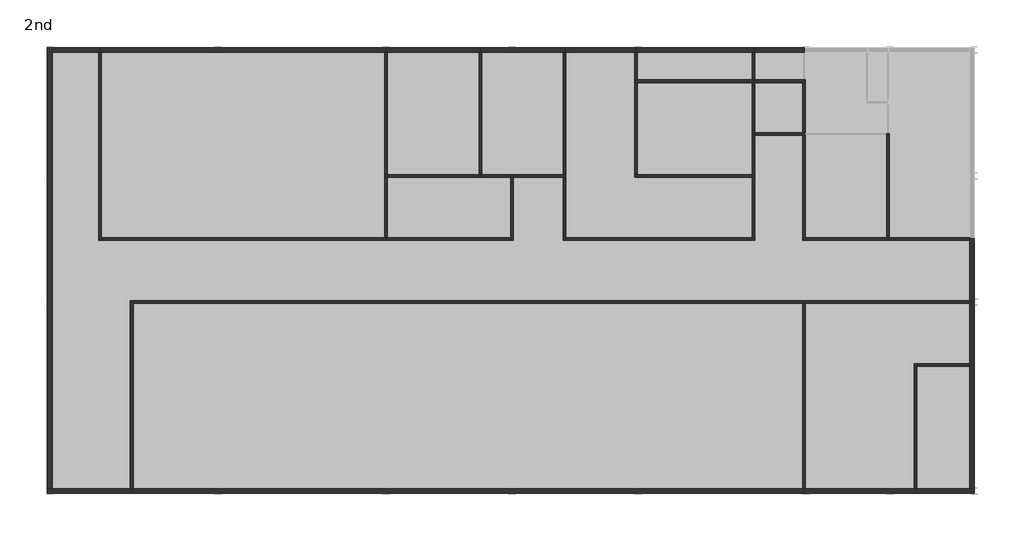
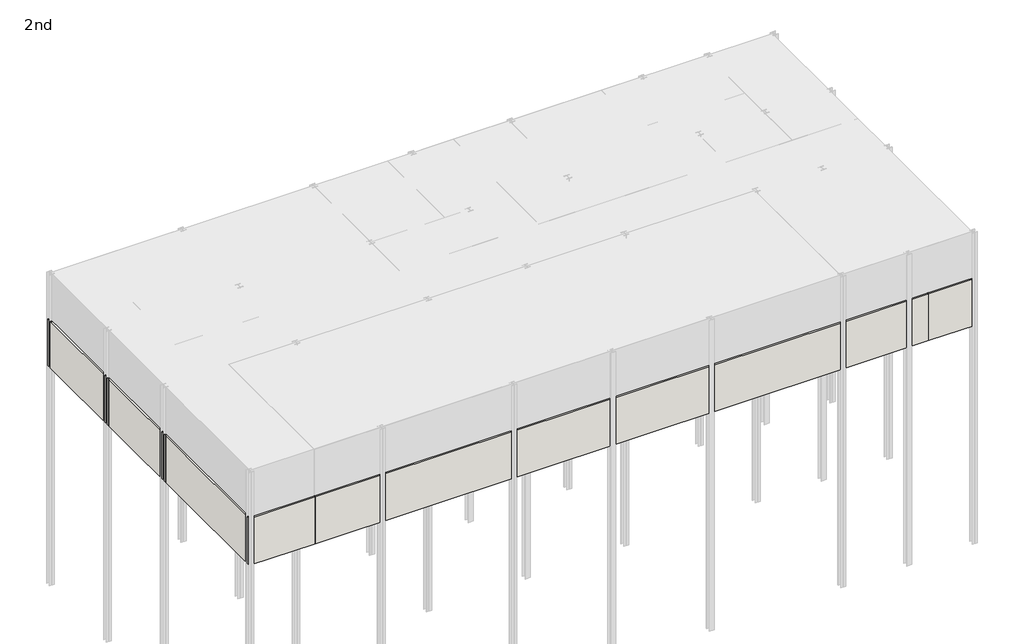
# One storey, part 1 of 3: 49 walls.
"""IFC4 building model written with IfcOpenShell, lengths in millimetres."""

from ifc_helpers import new_model, si_unit, frame, origin, place, context, project, spatial, polyline, outline, extrude, faceted_brep, element, save

model = new_model("IFC4")

# Units and contexts
model_context = context("Model", 3, world=origin())
ifc_project = project(units=[si_unit("LENGTHUNIT", "METRE", prefix="MILLI")], contexts=[model_context])

# Site, building, storey
site = spatial("IfcSite", under=ifc_project)
building = spatial("IfcBuilding", under=site)
storey = spatial("IfcBuildingStorey", under=building, Name="2nd", Elevation=14000.0)

# Walls
placement = place(None, origin())
element("IfcWall", 1, ObjectType="Wall-Ext_215Bwk", at=placement, inside=storey, context=model_context, shape_type="Brep", body=[
    faceted_brep([(160014.1020501, 130908.2581198, 14000.0), (192014.1020501, 130908.2581198, 14000.0), (192014.1020501, 130908.2581198, 17000.0), (160014.1020501, 130908.2581198, 17000.0), (160014.1020501, 131123.2581198, 14000.0), (160014.1020501, 131123.2581198, 17000.0), (160076.6020501, 131123.2581198, 17000.0), (191951.6020501, 131123.2581198, 17000.0), (192014.1020501, 131123.2581198, 17000.0), (192014.1020501, 131123.2581198, 14000.0), (191951.6020501, 131123.2581198, 14000.0), (160076.6020501, 131123.2581198, 14000.0)], [[[0, 1, 2, 3]], [[4, 5, 6, 7, 8, 9, 10, 11]], [[1, 0, 4, 11, 10, 9]], [[2, 1, 9, 8]], [[3, 2, 8, 7, 6, 5]], [[0, 3, 5, 4]]]),
])
element("IfcWall", 2, ObjectType="Wall-Ext_215Bwk", at=placement, inside=storey, context=model_context, shape_type="Brep", body=[
    faceted_brep([(172114.1020501, 152123.2581198, 14000.0), (158514.1020501, 152123.2581198, 14000.0), (158514.1020501, 152123.2581198, 17000.0), (172114.1020501, 152123.2581198, 17000.0), (172114.1020501, 151908.2581198, 14000.0), (172114.1020501, 151908.2581198, 17000.0), (172051.6020501, 151908.2581198, 17000.0), (158576.6020501, 151908.2581198, 17000.0), (158514.1020501, 151908.2581198, 17000.0), (158514.1020501, 151908.2581198, 14000.0), (158576.6020501, 151908.2581198, 14000.0), (172051.6020501, 151908.2581198, 14000.0)], [[[0, 1, 2, 3]], [[4, 5, 6, 7, 8, 9, 10, 11]], [[1, 0, 4, 11, 10, 9]], [[2, 1, 9, 8]], [[3, 2, 8, 7, 6, 5]], [[0, 3, 5, 4]]]),
])
element("IfcWall", 3, ObjectType="Wall-Ext_215Bwk", at=placement, inside=storey, context=model_context, shape_type="Brep", body=[
    faceted_brep([(176614.1020501, 152123.2581198, 14000.0), (172114.1020501, 152123.2581198, 14000.0), (172114.1020501, 152123.2581198, 17000.0), (176614.1020501, 152123.2581198, 17000.0), (176614.1020501, 151908.2581198, 14000.0), (176614.1020501, 151908.2581198, 17000.0), (176551.6020501, 151908.2581198, 17000.0), (172176.6020501, 151908.2581198, 17000.0), (172114.1020501, 151908.2581198, 17000.0), (172114.1020501, 151908.2581198, 14000.0), (172176.6020501, 151908.2581198, 14000.0), (176551.6020501, 151908.2581198, 14000.0)], [[[0, 1, 2, 3]], [[4, 5, 6, 7, 8, 9, 10, 11]], [[1, 0, 4, 11, 10, 9]], [[2, 1, 9, 8]], [[3, 2, 8, 7, 6, 5]], [[0, 3, 5, 4]]]),
])
element("IfcWall", 4, ObjectType="Wall-Ext_215Bwk", at=placement, inside=storey, context=model_context, shape_type="Brep", body=[
    faceted_brep([(180614.1020501, 152123.2581198, 14000.0), (176614.1020501, 152123.2581198, 14000.0), (176614.1020501, 152123.2581198, 17000.0), (180614.1020501, 152123.2581198, 17000.0), (180614.1020501, 151908.2581198, 14000.0), (180614.1020501, 151908.2581198, 17000.0), (180551.6020501, 151908.2581198, 17000.0), (176676.6020501, 151908.2581198, 17000.0), (176614.1020501, 151908.2581198, 17000.0), (176614.1020501, 151908.2581198, 14000.0), (176676.6020501, 151908.2581198, 14000.0), (180551.6020501, 151908.2581198, 14000.0)], [[[0, 1, 2, 3]], [[4, 5, 6, 7, 8, 9, 10, 11]], [[1, 0, 4, 11, 10, 9]], [[2, 1, 9, 8]], [[3, 2, 8, 7, 6, 5]], [[0, 3, 5, 4]]]),
])
element("IfcWall", 5, ObjectType="Wall-Ext_215Bwk", at=placement, inside=storey, context=model_context, shape_type="Brep", body=[
    faceted_brep([(192014.1020501, 152123.2581198, 14000.0), (189614.1020501, 152123.2581198, 14000.0), (189614.1020501, 152123.2581198, 17000.0), (192014.1020501, 152123.2581198, 17000.0), (192014.1020501, 151908.2581198, 14000.0), (192014.1020501, 151908.2581198, 17000.0), (191951.6020501, 151908.2581198, 17000.0), (189676.6020501, 151908.2581198, 17000.0), (189614.1020501, 151908.2581198, 17000.0), (189614.1020501, 151908.2581198, 14000.0), (189676.6020501, 151908.2581198, 14000.0), (191951.6020501, 151908.2581198, 14000.0)], [[[0, 1, 2, 3]], [[4, 5, 6, 7, 8, 9, 10, 11]], [[1, 0, 4, 11, 10, 9]], [[2, 1, 9, 8]], [[3, 2, 8, 7, 6, 5]], [[0, 3, 5, 4]]]),
])
element("IfcWall", 6, ObjectType="Wall-Ext_215Bwk", at=placement, inside=storey, context=model_context, shape_type="Brep", body=[
    faceted_brep([(200121.6020501, 140015.7581198, 14000.0), (200121.6020501, 143015.7581198, 14000.0), (200121.6020501, 143015.7581198, 17000.0), (200121.6020501, 140015.7581198, 17000.0), (199906.6020501, 140015.7581198, 14000.0), (199906.6020501, 140015.7581198, 17000.0), (199906.6020501, 140078.2581198, 17000.0), (199906.6020501, 142953.2581198, 17000.0), (199906.6020501, 143015.7581198, 17000.0), (199906.6020501, 143015.7581198, 14000.0), (199906.6020501, 142953.2581198, 14000.0), (199906.6020501, 140078.2581198, 14000.0)], [[[0, 1, 2, 3]], [[4, 5, 6, 7, 8, 9, 10, 11]], [[1, 0, 4, 11, 10, 9]], [[2, 1, 9, 8]], [[3, 2, 8, 7, 6, 5]], [[0, 3, 5, 4]]]),
])
element("IfcWall", 7, ObjectType="Wall-Ext_215Bwk", at=placement, inside=storey, context=model_context, shape_type="Brep", body=[
    faceted_brep([(158514.1020501, 152123.2581198, 14000.0), (156006.6020501, 152123.2581198, 14000.0), (156006.6020501, 152123.2581198, 17000.0), (158514.1020501, 152123.2581198, 17000.0), (158514.1020501, 151908.2581198, 14000.0), (158514.1020501, 151908.2581198, 17000.0), (158451.6020501, 151908.2581198, 17000.0), (156221.6020501, 151908.2581198, 17000.0), (156006.6020501, 151908.2581198, 17000.0), (156006.6020501, 151908.2581198, 14000.0), (156221.6020501, 151908.2581198, 14000.0), (158451.6020501, 151908.2581198, 14000.0)], [[[0, 1, 2, 3]], [[4, 5, 6, 7, 8, 9, 10, 11]], [[1, 0, 4, 11, 10, 9]], [[3, 2, 8, 7, 6, 5]], [[0, 3, 5, 4]], [[2, 1, 9, 8]]]),
])
element("IfcWall", 8, ObjectType="Wall-Ext_215Bwk", at=placement, inside=storey, context=model_context, shape_type="SweptSolid", body=[
    extrude(outline(polyline([(156006.6020501, 131123.2581198), (156006.6020501, 151908.2581198), (156221.6020501, 151908.2581198), (156221.6020501, 131123.2581198), (156006.6020501, 131123.2581198)])), frame((0.0, 0.0, 14000.0), z_axis=(0.0, 0.0, 1.0), x_axis=(1.0, 0.0, 0.0)), (0.0, 0.0, 1.0), 3000.0),
])
element("IfcWall", 9, ObjectType="Wall-Ext_215Bwk", at=placement, inside=storey, context=model_context, shape_type="Brep", body=[
    faceted_brep([(156006.6020501, 130908.2581198, 14000.0), (160014.1020501, 130908.2581198, 14000.0), (160014.1020501, 130908.2581198, 17000.0), (156006.6020501, 130908.2581198, 17000.0), (156006.6020501, 131123.2581198, 14000.0), (156006.6020501, 131123.2581198, 17000.0), (156221.6020501, 131123.2581198, 17000.0), (159951.6020501, 131123.2581198, 17000.0), (160014.1020501, 131123.2581198, 17000.0), (160014.1020501, 131123.2581198, 14000.0), (159951.6020501, 131123.2581198, 14000.0), (156221.6020501, 131123.2581198, 14000.0)], [[[0, 1, 2, 3]], [[4, 5, 6, 7, 8, 9, 10, 11]], [[1, 0, 4, 11, 10, 9]], [[2, 1, 9, 8]], [[3, 2, 8, 7, 6, 5]], [[0, 3, 5, 4]]]),
])
element("IfcWall", 10, ObjectType="Wall-Ext_215Bwk", at=placement, inside=storey, context=model_context, shape_type="Brep", body=[
    faceted_brep([(189614.1020501, 152123.2581198, 14000.0), (184014.1020501, 152123.2581198, 14000.0), (184014.1020501, 152123.2581198, 17000.0), (189614.1020501, 152123.2581198, 17000.0), (189614.1020501, 151908.2581198, 14000.0), (189614.1020501, 151908.2581198, 17000.0), (189551.6020501, 151908.2581198, 17000.0), (184076.6020501, 151908.2581198, 17000.0), (184014.1020501, 151908.2581198, 17000.0), (184014.1020501, 151908.2581198, 14000.0), (184076.6020501, 151908.2581198, 14000.0), (189551.6020501, 151908.2581198, 14000.0)], [[[0, 1, 2, 3]], [[4, 5, 6, 7, 8, 9, 10, 11]], [[1, 0, 4, 11, 10, 9]], [[2, 1, 9, 8]], [[3, 2, 8, 7, 6, 5]], [[0, 3, 5, 4]]]),
])
element("IfcWall", 11, ObjectType="Wall-Ext_215Bwk", at=placement, inside=storey, context=model_context, shape_type="Brep", body=[
    faceted_brep([(184014.1020501, 152123.2581198, 14000.0), (180614.1020501, 152123.2581198, 14000.0), (180614.1020501, 152123.2581198, 17000.0), (184014.1020501, 152123.2581198, 17000.0), (184014.1020501, 151908.2581198, 14000.0), (184014.1020501, 151908.2581198, 17000.0), (183951.6020501, 151908.2581198, 17000.0), (180676.6020501, 151908.2581198, 17000.0), (180614.1020501, 151908.2581198, 17000.0), (180614.1020501, 151908.2581198, 14000.0), (180676.6020501, 151908.2581198, 14000.0), (183951.6020501, 151908.2581198, 14000.0)], [[[0, 1, 2, 3]], [[4, 5, 6, 7, 8, 9, 10, 11]], [[1, 0, 4, 11, 10, 9]], [[2, 1, 9, 8]], [[3, 2, 8, 7, 6, 5]], [[0, 3, 5, 4]]]),
])
element("IfcWall", 12, ObjectType="Wall-Ext_215Bwk", at=placement, inside=storey, context=model_context, shape_type="Brep", body=[
    faceted_brep([(192014.1020501, 130908.2581198, 14000.0), (197314.1020501, 130908.2581198, 14000.0), (197314.1020501, 130908.2581198, 17000.0), (192014.1020501, 130908.2581198, 17000.0), (192014.1020501, 131123.2581198, 14000.0), (192014.1020501, 131123.2581198, 17000.0), (192076.6020501, 131123.2581198, 17000.0), (197314.1020501, 131123.2581198, 17000.0), (197314.1020501, 131123.2581198, 14000.0), (192076.6020501, 131123.2581198, 14000.0)], [[[0, 1, 2, 3]], [[4, 5, 6, 7, 8, 9]], [[1, 0, 4, 9, 8]], [[2, 1, 8, 7]], [[3, 2, 7, 6, 5]], [[0, 3, 5, 4]]]),
])
element("IfcWall", 13, ObjectType="Wall-Ext_215Bwk", at=placement, inside=storey, context=model_context, shape_type="Brep", body=[
    faceted_brep([(200121.6020501, 137015.7581198, 14000.0), (200121.6020501, 140015.7581198, 14000.0), (200121.6020501, 140015.7581198, 17000.0), (200121.6020501, 137015.7581198, 17000.0), (199906.6020501, 137015.7581198, 14000.0), (199906.6020501, 137015.7581198, 17000.0), (199906.6020501, 137078.2581198, 17000.0), (199906.6020501, 139953.2581198, 17000.0), (199906.6020501, 140015.7581198, 17000.0), (199906.6020501, 140015.7581198, 14000.0), (199906.6020501, 139953.2581198, 14000.0), (199906.6020501, 137078.2581198, 14000.0)], [[[0, 1, 2, 3]], [[4, 5, 6, 7, 8, 9, 10, 11]], [[1, 0, 4, 11, 10, 9]], [[2, 1, 9, 8]], [[3, 2, 8, 7, 6, 5]], [[0, 3, 5, 4]]]),
])
element("IfcWall", 14, ObjectType="Wall-Ext_215Bwk", at=placement, inside=storey, context=model_context, shape_type="Brep", body=[
    faceted_brep([(200121.6020501, 131123.2581198, 14000.0), (200121.6020501, 137015.7581198, 14000.0), (200121.6020501, 137015.7581198, 17000.0), (200121.6020501, 131123.2581198, 17000.0), (199906.6020501, 131123.2581198, 14000.0), (199906.6020501, 131123.2581198, 17000.0), (199906.6020501, 136953.2581198, 17000.0), (199906.6020501, 137015.7581198, 17000.0), (199906.6020501, 137015.7581198, 14000.0), (199906.6020501, 136953.2581198, 14000.0)], [[[0, 1, 2, 3]], [[4, 5, 6, 7, 8, 9]], [[1, 0, 4, 9, 8]], [[2, 1, 8, 7]], [[3, 2, 7, 6, 5]], [[0, 3, 5, 4]]]),
])
element("IfcWall", 15, ObjectType="Wall-Ext_215Bwk", at=placement, inside=storey, context=model_context, shape_type="Brep", body=[
    faceted_brep([(197314.1020501, 130908.2581198, 14000.0), (200121.6020501, 130908.2581198, 14000.0), (200121.6020501, 130908.2581198, 17000.0), (197314.1020501, 130908.2581198, 17000.0), (197314.1020501, 131123.2581198, 14000.0), (197314.1020501, 131123.2581198, 17000.0), (199906.6020501, 131123.2581198, 17000.0), (200121.6020501, 131123.2581198, 17000.0), (200121.6020501, 131123.2581198, 14000.0), (199906.6020501, 131123.2581198, 14000.0)], [[[0, 1, 2, 3]], [[4, 5, 6, 7, 8, 9]], [[1, 0, 4, 9, 8]], [[3, 2, 7, 6, 5]], [[0, 3, 5, 4]], [[2, 1, 8, 7]]]),
])
element("IfcWall", 16, ObjectType="Wall-Int_12P-100Blk-12P", at=placement, inside=storey, context=model_context, shape_type="SweptSolid", body=[
    extrude(outline(polyline([(160076.6020501, 140078.2581198), (191951.6020501, 140078.2581198), (191951.6020501, 139953.2581198), (160076.6020501, 139953.2581198), (160076.6020501, 140078.2581198)])), frame((0.0, 0.0, 14000.0), z_axis=(0.0, 0.0, 1.0), x_axis=(1.0, 0.0, 0.0)), (0.0, 0.0, 1.0), 3000.0),
])
element("IfcWall", 17, ObjectType="Wall-Int_12P-100Blk-12P", at=placement, inside=storey, context=model_context, shape_type="Brep", body=[
    faceted_brep([(159951.6020501, 140078.2581198, 14000.0), (159951.6020501, 131123.2581198, 14000.0), (159951.6020501, 131123.2581198, 17000.0), (159951.6020501, 140078.2581198, 17000.0), (160076.6020501, 140078.2581198, 14000.0), (160076.6020501, 140078.2581198, 17000.0), (160076.6020501, 139953.2581198, 17000.0), (160076.6020501, 131123.2581198, 17000.0), (160076.6020501, 131123.2581198, 14000.0), (160076.6020501, 139953.2581198, 14000.0), (160014.1020501, 131123.2581198, 14000.0), (160014.1020501, 131123.2581198, 17000.0)], [[[0, 1, 2, 3]], [[4, 5, 6, 7, 8, 9]], [[1, 0, 4, 9, 8, 10]], [[3, 2, 11, 7, 6, 5]], [[0, 3, 5, 4]], [[2, 1, 10, 8, 7, 11]]]),
])
element("IfcWall", 18, ObjectType="Wall-Int_12P-100Blk-12P", at=placement, inside=storey, context=model_context, shape_type="Brep", body=[
    faceted_brep([(192076.6020501, 131123.2581198, 14000.0), (192076.6020501, 139953.2581198, 14000.0), (192076.6020501, 140078.2581198, 14000.0), (192076.6020501, 140078.2581198, 17000.0), (192076.6020501, 139953.2581198, 17000.0), (192076.6020501, 131123.2581198, 17000.0), (191951.6020501, 131123.2581198, 14000.0), (191951.6020501, 131123.2581198, 17000.0), (191951.6020501, 139953.2581198, 17000.0), (191951.6020501, 140078.2581198, 17000.0), (191951.6020501, 140078.2581198, 14000.0), (191951.6020501, 139953.2581198, 14000.0), (192014.1020501, 131123.2581198, 14000.0), (192014.1020501, 131123.2581198, 17000.0)], [[[0, 1, 2, 3, 4, 5]], [[6, 7, 8, 9, 10, 11]], [[2, 1, 0, 12, 6, 11, 10]], [[5, 4, 3, 9, 8, 7, 13]], [[3, 2, 10, 9]], [[0, 5, 13, 7, 6, 12]]]),
])
element("IfcWall", 19, ObjectType="Wall-Int_12P-100Blk-12P", at=placement, inside=storey, context=model_context, shape_type="Brep", body=[
    faceted_brep([(158451.6020501, 151908.2581198, 14000.0), (158451.6020501, 142953.2581198, 14000.0), (158451.6020501, 142953.2581198, 17000.0), (158451.6020501, 151908.2581198, 17000.0), (158576.6020501, 151908.2581198, 14000.0), (158576.6020501, 151908.2581198, 17000.0), (158576.6020501, 143078.2581198, 17000.0), (158576.6020501, 142953.2581198, 17000.0), (158576.6020501, 142953.2581198, 14000.0), (158576.6020501, 143078.2581198, 14000.0), (158514.1020501, 151908.2581198, 14000.0), (158514.1020501, 151908.2581198, 17000.0)], [[[0, 1, 2, 3]], [[4, 5, 6, 7, 8, 9]], [[1, 0, 10, 4, 9, 8]], [[3, 2, 7, 6, 5, 11]], [[0, 3, 11, 5, 4, 10]], [[2, 1, 8, 7]]]),
])
element("IfcWall", 20, ObjectType="Wall-Int_12P-100Blk-12P", at=placement, inside=storey, context=model_context, shape_type="Brep", body=[
    faceted_brep([(158576.6020501, 142953.2581198, 14000.0), (172114.1020501, 142953.2581198, 14000.0), (172114.1020501, 142953.2581198, 17000.0), (158576.6020501, 142953.2581198, 17000.0), (158576.6020501, 143078.2581198, 14000.0), (158576.6020501, 143078.2581198, 17000.0), (172051.6020501, 143078.2581198, 17000.0), (172114.1020501, 143078.2581198, 17000.0), (172114.1020501, 143078.2581198, 14000.0), (172051.6020501, 143078.2581198, 14000.0)], [[[0, 1, 2, 3]], [[4, 5, 6, 7, 8, 9]], [[1, 0, 4, 9, 8]], [[2, 1, 8, 7]], [[3, 2, 7, 6, 5]], [[0, 3, 5, 4]]]),
])
element("IfcWall", 21, ObjectType="Wall-Int_12P-100Blk-12P", at=placement, inside=storey, context=model_context, shape_type="Brep", body=[
    faceted_brep([(172176.6020501, 143078.2581198, 14000.0), (172176.6020501, 145953.2581198, 14000.0), (172176.6020501, 145953.2581198, 17000.0), (172176.6020501, 143078.2581198, 17000.0), (172051.6020501, 143078.2581198, 14000.0), (172051.6020501, 143078.2581198, 17000.0), (172051.6020501, 145953.2581198, 17000.0), (172051.6020501, 145953.2581198, 14000.0), (172114.1020501, 143078.2581198, 14000.0), (172114.1020501, 143078.2581198, 17000.0)], [[[0, 1, 2, 3]], [[4, 5, 6, 7]], [[1, 0, 8, 4, 7]], [[3, 2, 6, 5, 9]], [[0, 3, 9, 5, 4, 8]], [[2, 1, 7, 6]]]),
])
element("IfcWall", 22, ObjectType="Wall-Int_12P-100Blk-12P", at=placement, inside=storey, context=model_context, shape_type="Brep", body=[
    faceted_brep([(172176.6020501, 146078.2581198, 14000.0), (172176.6020501, 151908.2581198, 14000.0), (172176.6020501, 151908.2581198, 17000.0), (172176.6020501, 146078.2581198, 17000.0), (172051.6020501, 146078.2581198, 14000.0), (172051.6020501, 146078.2581198, 17000.0), (172051.6020501, 151908.2581198, 17000.0), (172051.6020501, 151908.2581198, 14000.0), (172114.1020501, 151908.2581198, 14000.0), (172114.1020501, 151908.2581198, 17000.0)], [[[0, 1, 2, 3]], [[4, 5, 6, 7]], [[1, 0, 4, 7, 8]], [[3, 2, 9, 6, 5]], [[2, 1, 8, 7, 6, 9]], [[0, 3, 5, 4]]]),
])
element("IfcWall", 23, ObjectType="Wall-Int_12P-100Blk-12P", at=placement, inside=storey, context=model_context, shape_type="Brep", body=[
    faceted_brep([(172051.6020501, 145953.2581198, 14000.0), (172176.6020501, 145953.2581198, 14000.0), (176614.1020501, 145953.2581198, 14000.0), (176614.1020501, 145953.2581198, 17000.0), (172176.6020501, 145953.2581198, 17000.0), (172051.6020501, 145953.2581198, 17000.0), (172051.6020501, 146078.2581198, 14000.0), (172051.6020501, 146078.2581198, 17000.0), (172176.6020501, 146078.2581198, 17000.0), (176551.6020501, 146078.2581198, 17000.0), (176614.1020501, 146078.2581198, 17000.0), (176614.1020501, 146078.2581198, 14000.0), (176551.6020501, 146078.2581198, 14000.0), (172176.6020501, 146078.2581198, 14000.0)], [[[0, 1, 2, 3, 4, 5]], [[6, 7, 8, 9, 10, 11, 12, 13]], [[2, 1, 0, 6, 13, 12, 11]], [[3, 2, 11, 10]], [[5, 4, 3, 10, 9, 8, 7]], [[0, 5, 7, 6]]]),
])
element("IfcWall", 24, ObjectType="Wall-Int_12P-100Blk-12P", at=placement, inside=storey, context=model_context, shape_type="Brep", body=[
    faceted_brep([(176676.6020501, 146078.2581198, 14000.0), (176676.6020501, 151908.2581198, 14000.0), (176676.6020501, 151908.2581198, 17000.0), (176676.6020501, 146078.2581198, 17000.0), (176551.6020501, 146078.2581198, 14000.0), (176551.6020501, 146078.2581198, 17000.0), (176551.6020501, 151908.2581198, 17000.0), (176551.6020501, 151908.2581198, 14000.0), (176614.1020501, 146078.2581198, 14000.0), (176614.1020501, 151908.2581198, 14000.0), (176614.1020501, 151908.2581198, 17000.0), (176614.1020501, 146078.2581198, 17000.0)], [[[0, 1, 2, 3]], [[4, 5, 6, 7]], [[1, 0, 8, 4, 7, 9]], [[3, 2, 10, 6, 5, 11]], [[2, 1, 9, 7, 6, 10]], [[0, 3, 11, 5, 4, 8]]]),
])
element("IfcWall", 25, ObjectType="Wall-Int_12P-100Blk-12P", at=placement, inside=storey, context=model_context, shape_type="Brep", body=[
    faceted_brep([(191951.6020501, 147953.2581198, 14000.0), (191951.6020501, 143078.2581198, 14000.0), (191951.6020501, 143078.2581198, 17000.0), (191951.6020501, 147953.2581198, 17000.0), (192076.6020501, 147953.2581198, 14000.0), (192076.6020501, 147953.2581198, 17000.0), (192076.6020501, 143078.2581198, 17000.0), (192076.6020501, 143078.2581198, 14000.0), (192014.1020501, 147953.2581198, 14000.0), (192014.1020501, 147953.2581198, 17000.0)], [[[0, 1, 2, 3]], [[4, 5, 6, 7]], [[1, 0, 8, 4, 7]], [[3, 2, 6, 5, 9]], [[0, 3, 9, 5, 4, 8]], [[2, 1, 7, 6]]]),
])
element("IfcWall", 26, ObjectType="Wall-Int_12P-100Blk-12P", at=placement, inside=storey, context=model_context, shape_type="Brep", body=[
    faceted_brep([(191951.6020501, 142953.2581198, 14000.0), (196014.1020501, 142953.2581198, 14000.0), (196014.1020501, 142953.2581198, 17000.0), (191951.6020501, 142953.2581198, 17000.0), (191951.6020501, 143078.2581198, 14000.0), (191951.6020501, 143078.2581198, 17000.0), (192076.6020501, 143078.2581198, 17000.0), (195951.6020501, 143078.2581198, 17000.0), (196014.1020501, 143078.2581198, 17000.0), (196014.1020501, 143078.2581198, 14000.0), (195951.6020501, 143078.2581198, 14000.0), (192076.6020501, 143078.2581198, 14000.0)], [[[0, 1, 2, 3]], [[4, 5, 6, 7, 8, 9, 10, 11]], [[1, 0, 4, 11, 10, 9]], [[2, 1, 9, 8]], [[3, 2, 8, 7, 6, 5]], [[0, 3, 5, 4]]]),
])
element("IfcWall", 27, ObjectType="Wall-Int_12P-100Blk-12P", at=placement, inside=storey, context=model_context, shape_type="Brep", body=[
    faceted_brep([(196076.6020501, 143078.2581198, 14000.0), (196076.6020501, 148015.7581198, 14000.0), (196076.6020501, 148015.7581198, 17000.0), (196076.6020501, 143078.2581198, 17000.0), (195951.6020501, 143078.2581198, 14000.0), (195951.6020501, 143078.2581198, 17000.0), (195951.6020501, 147953.2581198, 17000.0), (195951.6020501, 148015.7581198, 17000.0), (195951.6020501, 148015.7581198, 14000.0), (195951.6020501, 147953.2581198, 14000.0), (196014.1020501, 143078.2581198, 14000.0), (196014.1020501, 143078.2581198, 17000.0)], [[[0, 1, 2, 3]], [[4, 5, 6, 7, 8, 9]], [[1, 0, 10, 4, 9, 8]], [[2, 1, 8, 7]], [[3, 2, 7, 6, 5, 11]], [[0, 3, 11, 5, 4, 10]]]),
])
element("IfcWall", 28, ObjectType="Wall-Int_12P-100Blk-12P", at=placement, inside=storey, context=model_context, shape_type="Brep", body=[
    faceted_brep([(196014.1020501, 142953.2581198, 14000.0), (199906.6020501, 142953.2581198, 14000.0), (199906.6020501, 142953.2581198, 17000.0), (196014.1020501, 142953.2581198, 17000.0), (196014.1020501, 143078.2581198, 14000.0), (196014.1020501, 143078.2581198, 17000.0), (196076.6020501, 143078.2581198, 17000.0), (199906.6020501, 143078.2581198, 17000.0), (199906.6020501, 143078.2581198, 14000.0), (196076.6020501, 143078.2581198, 14000.0), (199906.6020501, 143015.7581198, 14000.0), (199906.6020501, 143015.7581198, 17000.0)], [[[0, 1, 2, 3]], [[4, 5, 6, 7, 8, 9]], [[1, 0, 4, 9, 8, 10]], [[3, 2, 11, 7, 6, 5]], [[0, 3, 5, 4]], [[2, 1, 10, 8, 7, 11]]]),
])
element("IfcWall", 29, ObjectType="Wall-Int_12P-100Blk-12P", at=placement, inside=storey, context=model_context, shape_type="Brep", body=[
    faceted_brep([(176614.1020501, 145953.2581198, 14000.0), (178051.6020501, 145953.2581198, 14000.0), (178051.6020501, 145953.2581198, 17000.0), (176614.1020501, 145953.2581198, 17000.0), (176614.1020501, 146078.2581198, 14000.0), (176614.1020501, 146078.2581198, 17000.0), (176676.6020501, 146078.2581198, 17000.0), (178051.6020501, 146078.2581198, 17000.0), (178051.6020501, 146078.2581198, 14000.0), (176676.6020501, 146078.2581198, 14000.0)], [[[0, 1, 2, 3]], [[4, 5, 6, 7, 8, 9]], [[1, 0, 4, 9, 8]], [[3, 2, 7, 6, 5]], [[0, 3, 5, 4]], [[2, 1, 8, 7]]]),
])
element("IfcWall", 30, ObjectType="Wall-Int_12P-100Blk-12P", at=placement, inside=storey, context=model_context, shape_type="Brep", body=[
    faceted_brep([(178176.6020501, 145953.2581198, 14000.0), (180551.6020501, 145953.2581198, 14000.0), (180676.6020501, 145953.2581198, 14000.0), (180676.6020501, 145953.2581198, 17000.0), (180551.6020501, 145953.2581198, 17000.0), (178176.6020501, 145953.2581198, 17000.0), (178176.6020501, 146078.2581198, 14000.0), (178176.6020501, 146078.2581198, 17000.0), (180551.6020501, 146078.2581198, 17000.0), (180676.6020501, 146078.2581198, 17000.0), (180676.6020501, 146078.2581198, 14000.0), (180551.6020501, 146078.2581198, 14000.0)], [[[0, 1, 2, 3, 4, 5]], [[6, 7, 8, 9, 10, 11]], [[2, 1, 0, 6, 11, 10]], [[5, 4, 3, 9, 8, 7]], [[3, 2, 10, 9]], [[0, 5, 7, 6]]]),
])
element("IfcWall", 31, ObjectType="Wall-Int_12P-100Blk-12P", at=placement, inside=storey, context=model_context, shape_type="Brep", body=[
    faceted_brep([(180676.6020501, 146078.2581198, 14000.0), (180676.6020501, 151908.2581198, 14000.0), (180676.6020501, 151908.2581198, 17000.0), (180676.6020501, 146078.2581198, 17000.0), (180551.6020501, 146078.2581198, 14000.0), (180551.6020501, 146078.2581198, 17000.0), (180551.6020501, 151908.2581198, 17000.0), (180551.6020501, 151908.2581198, 14000.0), (180614.1020501, 151908.2581198, 14000.0), (180614.1020501, 151908.2581198, 17000.0)], [[[0, 1, 2, 3]], [[4, 5, 6, 7]], [[1, 0, 4, 7, 8]], [[3, 2, 9, 6, 5]], [[2, 1, 8, 7, 6, 9]], [[0, 3, 5, 4]]]),
])
element("IfcWall", 32, ObjectType="Wall-Int_12P-100Blk-12P", at=placement, inside=storey, context=model_context, shape_type="Brep", body=[
    faceted_brep([(172114.1020501, 142953.2581198, 14000.0), (178051.6020501, 142953.2581198, 14000.0), (178051.6020501, 142953.2581198, 17000.0), (172114.1020501, 142953.2581198, 17000.0), (172114.1020501, 143078.2581198, 14000.0), (172114.1020501, 143078.2581198, 17000.0), (172176.6020501, 143078.2581198, 17000.0), (178051.6020501, 143078.2581198, 17000.0), (178051.6020501, 143078.2581198, 14000.0), (172176.6020501, 143078.2581198, 14000.0)], [[[0, 1, 2, 3]], [[4, 5, 6, 7, 8, 9]], [[1, 0, 4, 9, 8]], [[3, 2, 7, 6, 5]], [[0, 3, 5, 4]], [[2, 1, 8, 7]]]),
])
element("IfcWall", 33, ObjectType="Wall-Int_12P-100Blk-12P", at=placement, inside=storey, context=model_context, shape_type="Brep", body=[
    faceted_brep([(178176.6020501, 142953.2581198, 14000.0), (178176.6020501, 145953.2581198, 14000.0), (178176.6020501, 146078.2581198, 14000.0), (178176.6020501, 146078.2581198, 17000.0), (178176.6020501, 145953.2581198, 17000.0), (178176.6020501, 142953.2581198, 17000.0), (178051.6020501, 142953.2581198, 14000.0), (178051.6020501, 142953.2581198, 17000.0), (178051.6020501, 143078.2581198, 17000.0), (178051.6020501, 145953.2581198, 17000.0), (178051.6020501, 146078.2581198, 17000.0), (178051.6020501, 146078.2581198, 14000.0), (178051.6020501, 145953.2581198, 14000.0), (178051.6020501, 143078.2581198, 14000.0)], [[[0, 1, 2, 3, 4, 5]], [[6, 7, 8, 9, 10, 11, 12, 13]], [[2, 1, 0, 6, 13, 12, 11]], [[5, 4, 3, 10, 9, 8, 7]], [[0, 5, 7, 6]], [[3, 2, 11, 10]]]),
])
element("IfcWall", 34, ObjectType="Wall-Int_12P-100Blk-12P", at=placement, inside=storey, context=model_context, shape_type="Brep", body=[
    faceted_brep([(189551.6020501, 151908.2581198, 14000.0), (189551.6020501, 150578.2581198, 14000.0), (189551.6020501, 150578.2581198, 17000.0), (189551.6020501, 151908.2581198, 17000.0), (189676.6020501, 151908.2581198, 14000.0), (189676.6020501, 151908.2581198, 17000.0), (189676.6020501, 150578.2581198, 17000.0), (189676.6020501, 150578.2581198, 14000.0), (189614.1020501, 151908.2581198, 14000.0), (189614.1020501, 150578.2581198, 14000.0), (189614.1020501, 150578.2581198, 17000.0), (189614.1020501, 151908.2581198, 17000.0)], [[[0, 1, 2, 3]], [[4, 5, 6, 7]], [[1, 0, 8, 4, 7, 9]], [[3, 2, 10, 6, 5, 11]], [[0, 3, 11, 5, 4, 8]], [[2, 1, 9, 7, 6, 10]]]),
])
element("IfcWall", 35, ObjectType="Wall-Int_12P-100Blk-12P", at=placement, inside=storey, context=model_context, shape_type="Brep", body=[
    faceted_brep([(189614.1020501, 150453.2581198, 14000.0), (189676.6020501, 150453.2581198, 14000.0), (191951.6020501, 150453.2581198, 14000.0), (192076.6020501, 150453.2581198, 14000.0), (192076.6020501, 150453.2581198, 17000.0), (191951.6020501, 150453.2581198, 17000.0), (189676.6020501, 150453.2581198, 17000.0), (189614.1020501, 150453.2581198, 17000.0), (189614.1020501, 150578.2581198, 14000.0), (189614.1020501, 150578.2581198, 17000.0), (189676.6020501, 150578.2581198, 17000.0), (191951.6020501, 150578.2581198, 17000.0), (192076.6020501, 150578.2581198, 17000.0), (192076.6020501, 150578.2581198, 14000.0), (191951.6020501, 150578.2581198, 14000.0), (189676.6020501, 150578.2581198, 14000.0)], [[[0, 1, 2, 3, 4, 5, 6, 7]], [[8, 9, 10, 11, 12, 13, 14, 15]], [[3, 2, 1, 0, 8, 15, 14, 13]], [[7, 6, 5, 4, 12, 11, 10, 9]], [[0, 7, 9, 8]], [[4, 3, 13, 12]]]),
])
element("IfcWall", 36, ObjectType="Wall-Int_12P-100Blk-12P", at=placement, inside=storey, context=model_context, shape_type="Brep", body=[
    faceted_brep([(192076.6020501, 139953.2581198, 14000.0), (199906.6020501, 139953.2581198, 14000.0), (199906.6020501, 139953.2581198, 17000.0), (192076.6020501, 139953.2581198, 17000.0), (192076.6020501, 140078.2581198, 14000.0), (192076.6020501, 140078.2581198, 17000.0), (199906.6020501, 140078.2581198, 17000.0), (199906.6020501, 140078.2581198, 14000.0), (199906.6020501, 140015.7581198, 14000.0), (199906.6020501, 140015.7581198, 17000.0)], [[[0, 1, 2, 3]], [[4, 5, 6, 7]], [[1, 0, 4, 7, 8]], [[3, 2, 9, 6, 5]], [[0, 3, 5, 4]], [[2, 1, 8, 7, 6, 9]]]),
])
element("IfcWall", 37, ObjectType="Wall-Int_12P-100Blk-12P", at=placement, inside=storey, context=model_context, shape_type="Brep", body=[
    faceted_brep([(192014.1020501, 148078.2581198, 14000.0), (191951.6020501, 148078.2581198, 14000.0), (189614.1020501, 148078.2581198, 14000.0), (189614.1020501, 148078.2581198, 17000.0), (191951.6020501, 148078.2581198, 17000.0), (192014.1020501, 148078.2581198, 17000.0), (192014.1020501, 147953.2581198, 14000.0), (192014.1020501, 147953.2581198, 17000.0), (191951.6020501, 147953.2581198, 17000.0), (189614.1020501, 147953.2581198, 17000.0), (189614.1020501, 147953.2581198, 14000.0), (191951.6020501, 147953.2581198, 14000.0)], [[[0, 1, 2, 3, 4, 5]], [[6, 7, 8, 9, 10, 11]], [[2, 1, 0, 6, 11, 10]], [[3, 2, 10, 9]], [[5, 4, 3, 9, 8, 7]], [[0, 5, 7, 6]]]),
])
element("IfcWall", 38, ObjectType="Wall-Int_12P-100Blk-12P", at=placement, inside=storey, context=model_context, shape_type="SweptSolid", body=[
    extrude(outline(polyline([(189551.6020501, 146015.7581198), (189551.6020501, 148015.7581198), (189676.6020501, 148015.7581198), (189676.6020501, 146015.7581198), (189551.6020501, 146015.7581198)])), frame((0.0, 0.0, 14000.0), z_axis=(0.0, 0.0, 1.0), x_axis=(1.0, 0.0, 0.0)), (0.0, 0.0, 1.0), 3000.0),
])
element("IfcWall", 39, ObjectType="Wall-Int_12P-100Blk-12P", at=placement, inside=storey, context=model_context, shape_type="SweptSolid", body=[
    extrude(outline(polyline([(189551.6020501, 143078.2581198), (189551.6020501, 146015.7581198), (189676.6020501, 146015.7581198), (189676.6020501, 143078.2581198), (189551.6020501, 143078.2581198)])), frame((0.0, 0.0, 14000.0), z_axis=(0.0, 0.0, 1.0), x_axis=(1.0, 0.0, 0.0)), (0.0, 0.0, 1.0), 3000.0),
])
element("IfcWall", 40, ObjectType="Wall-Int_12P-100Blk-12P", at=placement, inside=storey, context=model_context, shape_type="Brep", body=[
    faceted_brep([(189676.6020501, 143078.2581198, 14000.0), (189551.6020501, 143078.2581198, 14000.0), (180676.6020501, 143078.2581198, 14000.0), (180551.6020501, 143078.2581198, 14000.0), (180551.6020501, 143078.2581198, 17000.0), (180676.6020501, 143078.2581198, 17000.0), (189551.6020501, 143078.2581198, 17000.0), (189676.6020501, 143078.2581198, 17000.0), (189676.6020501, 142953.2581198, 14000.0), (189676.6020501, 142953.2581198, 17000.0), (180551.6020501, 142953.2581198, 17000.0), (180551.6020501, 142953.2581198, 14000.0)], [[[0, 1, 2, 3, 4, 5, 6, 7]], [[8, 9, 10, 11]], [[3, 2, 1, 0, 8, 11]], [[7, 6, 5, 4, 10, 9]], [[0, 7, 9, 8]], [[4, 3, 11, 10]]]),
])
element("IfcWall", 41, ObjectType="Wall-Int_12P-100Blk-12P", at=placement, inside=storey, context=model_context, shape_type="SweptSolid", body=[
    extrude(outline(polyline([(180676.6020501, 145953.2581198), (180676.6020501, 143078.2581198), (180551.6020501, 143078.2581198), (180551.6020501, 145953.2581198), (180676.6020501, 145953.2581198)])), frame((0.0, 0.0, 14000.0), z_axis=(0.0, 0.0, 1.0), x_axis=(1.0, 0.0, 0.0)), (0.0, 0.0, 1.0), 3000.0),
])
element("IfcWall", 42, ObjectType="Wall-Int_12P-100Blk-12P", at=placement, inside=storey, context=model_context, shape_type="Brep", body=[
    faceted_brep([(189551.6020501, 150453.2581198, 14000.0), (189551.6020501, 148015.7581198, 14000.0), (189551.6020501, 148015.7581198, 17000.0), (189551.6020501, 150453.2581198, 17000.0), (189676.6020501, 150453.2581198, 14000.0), (189676.6020501, 150453.2581198, 17000.0), (189676.6020501, 148015.7581198, 17000.0), (189676.6020501, 148015.7581198, 14000.0), (189614.1020501, 150453.2581198, 14000.0), (189614.1020501, 150453.2581198, 17000.0)], [[[0, 1, 2, 3]], [[4, 5, 6, 7]], [[1, 0, 8, 4, 7]], [[2, 1, 7, 6]], [[3, 2, 6, 5, 9]], [[0, 3, 9, 5, 4, 8]]]),
])
element("IfcWall", 43, ObjectType="Wall-Int_12P-100Blk-12P", at=placement, inside=storey, context=model_context, shape_type="Brep", body=[
    faceted_brep([(192076.6020501, 148078.2581198, 14000.0), (192076.6020501, 150453.2581198, 14000.0), (192076.6020501, 150453.2581198, 17000.0), (192076.6020501, 148078.2581198, 17000.0), (191951.6020501, 148078.2581198, 14000.0), (191951.6020501, 148078.2581198, 17000.0), (191951.6020501, 150453.2581198, 17000.0), (191951.6020501, 150453.2581198, 14000.0), (192014.1020501, 148078.2581198, 14000.0), (192014.1020501, 148078.2581198, 17000.0)], [[[0, 1, 2, 3]], [[4, 5, 6, 7]], [[1, 0, 8, 4, 7]], [[3, 2, 6, 5, 9]], [[0, 3, 9, 5, 4, 8]], [[2, 1, 7, 6]]]),
])
element("IfcWall", 44, ObjectType="Wall-Int_12P-100Blk-12P", at=placement, inside=storey, context=model_context, shape_type="Brep", body=[
    faceted_brep([(183951.6020501, 151908.2581198, 14000.0), (183951.6020501, 150578.2581198, 14000.0), (183951.6020501, 150578.2581198, 17000.0), (183951.6020501, 151908.2581198, 17000.0), (184076.6020501, 151908.2581198, 14000.0), (184076.6020501, 151908.2581198, 17000.0), (184076.6020501, 150578.2581198, 17000.0), (184076.6020501, 150578.2581198, 14000.0), (184014.1020501, 151908.2581198, 14000.0), (184014.1020501, 151908.2581198, 17000.0)], [[[0, 1, 2, 3]], [[4, 5, 6, 7]], [[1, 0, 8, 4, 7]], [[3, 2, 6, 5, 9]], [[0, 3, 9, 5, 4, 8]], [[2, 1, 7, 6]]]),
])
element("IfcWall", 45, ObjectType="Wall-Int_12P-100Blk-12P", at=placement, inside=storey, context=model_context, shape_type="Brep", body=[
    faceted_brep([(183951.6020501, 150453.2581198, 14000.0), (184076.6020501, 150453.2581198, 14000.0), (189551.6020501, 150453.2581198, 14000.0), (189614.1020501, 150453.2581198, 14000.0), (189614.1020501, 150453.2581198, 17000.0), (189551.6020501, 150453.2581198, 17000.0), (184076.6020501, 150453.2581198, 17000.0), (183951.6020501, 150453.2581198, 17000.0), (183951.6020501, 150578.2581198, 14000.0), (183951.6020501, 150578.2581198, 17000.0), (184076.6020501, 150578.2581198, 17000.0), (189551.6020501, 150578.2581198, 17000.0), (189614.1020501, 150578.2581198, 17000.0), (189614.1020501, 150578.2581198, 14000.0), (189551.6020501, 150578.2581198, 14000.0), (184076.6020501, 150578.2581198, 14000.0)], [[[0, 1, 2, 3, 4, 5, 6, 7]], [[8, 9, 10, 11, 12, 13, 14, 15]], [[3, 2, 1, 0, 8, 15, 14, 13]], [[4, 3, 13, 12]], [[7, 6, 5, 4, 12, 11, 10, 9]], [[0, 7, 9, 8]]]),
])
element("IfcWall", 46, ObjectType="Wall-Int_12P-100Blk-12P", at=placement, inside=storey, context=model_context, shape_type="Brep", body=[
    faceted_brep([(189614.1020501, 146078.2581198, 14000.0), (184076.6020501, 146078.2581198, 14000.0), (183951.6020501, 146078.2581198, 14000.0), (183951.6020501, 146078.2581198, 17000.0), (184076.6020501, 146078.2581198, 17000.0), (189614.1020501, 146078.2581198, 17000.0), (189614.1020501, 145953.2581198, 14000.0), (189614.1020501, 145953.2581198, 17000.0), (183951.6020501, 145953.2581198, 17000.0), (183951.6020501, 145953.2581198, 14000.0)], [[[0, 1, 2, 3, 4, 5]], [[6, 7, 8, 9]], [[2, 1, 0, 6, 9]], [[5, 4, 3, 8, 7]], [[0, 5, 7, 6]], [[3, 2, 9, 8]]]),
])
element("IfcWall", 47, ObjectType="Wall-Int_12P-100Blk-12P", at=placement, inside=storey, context=model_context, shape_type="SweptSolid", body=[
    extrude(outline(polyline([(184076.6020501, 150453.2581198), (184076.6020501, 146078.2581198), (183951.6020501, 146078.2581198), (183951.6020501, 150453.2581198), (184076.6020501, 150453.2581198)])), frame((0.0, 0.0, 14000.0), z_axis=(0.0, 0.0, 1.0), x_axis=(1.0, 0.0, 0.0)), (0.0, 0.0, 1.0), 3000.0),
])
element("IfcWall", 48, ObjectType="Wall-Int_12P-100Blk-12P", at=placement, inside=storey, context=model_context, shape_type="SweptSolid", body=[
    extrude(outline(polyline([(197376.6020501, 136953.2581198), (197376.6020501, 131015.7581198), (197251.6020501, 131015.7581198), (197251.6020501, 136953.2581198), (197376.6020501, 136953.2581198)])), frame((0.0, 0.0, 14000.0), z_axis=(0.0, 0.0, 1.0), x_axis=(1.0, 0.0, 0.0)), (0.0, 0.0, 1.0), 3000.0),
])
element("IfcWall", 49, ObjectType="Wall-Int_12P-100Blk-12P", at=placement, inside=storey, context=model_context, shape_type="Brep", body=[
    faceted_brep([(197251.6020501, 136953.2581198, 14000.0), (197376.6020501, 136953.2581198, 14000.0), (199906.6020501, 136953.2581198, 14000.0), (199906.6020501, 136953.2581198, 17000.0), (197376.6020501, 136953.2581198, 17000.0), (197251.6020501, 136953.2581198, 17000.0), (197251.6020501, 137078.2581198, 14000.0), (197251.6020501, 137078.2581198, 17000.0), (199906.6020501, 137078.2581198, 17000.0), (199906.6020501, 137078.2581198, 14000.0), (199906.6020501, 137015.7581198, 14000.0), (199906.6020501, 137015.7581198, 17000.0)], [[[0, 1, 2, 3, 4, 5]], [[6, 7, 8, 9]], [[2, 1, 0, 6, 9, 10]], [[5, 4, 3, 11, 8, 7]], [[0, 5, 7, 6]], [[3, 2, 10, 9, 8, 11]]]),
])

save(model, "model.ifc")

# Revit data of these elements
# Project information
#   Project Issue Date = "Issue Date"
#   Project Status = "Project Status"
#   Client Name = "Owner"
#   Project Address = "Enter address here"
#   Project Name = "Project Name"
#   Project Number = "Project Number"
# Grids (mm)
#   "A": line (156114.102, 123537.292) -> (156114.102, 157930.913)
#   "B": line (164114.102, 123537.292) -> (164114.102, 157930.913)
#   "C": line (172114.102, 123537.292) -> (172114.102, 157930.913)
#   "D": line (178114.102, 123537.292) -> (178114.102, 157930.913)
#   "E": line (184114.102, 123537.292) -> (184114.102, 157930.913)
#   "F": line (192114.102, 123537.292) -> (192114.102, 157930.913)
#   "G": line (196114.102, 123537.292) -> (196114.102, 157930.913)
#   "8": line (145724.678, 152015.758) -> (209069.776, 152015.758)
#   "3": line (145724.678, 146015.758) -> (209069.776, 146015.758)
#   "2": line (145724.678, 140015.758) -> (209069.776, 140015.758)
#   "1": line (145724.678, 131015.758) -> (209069.776, 131015.758)
#   "H": line (200114.102, 123537.292) -> (200114.102, 157930.913)
# Type "Wall-Ext_215Bwk"
#   Keynote = "F10"
#   Layers, outside or top first: 215 mm "Brick, Common" (function 1)
# Type "Wall-Int_12P-100Blk-12P"
#   Layers, outside or top first: 12.5 mm "Plaster" (function 5); 100 mm "Concrete Masonry Units" (function 1); 12.5 mm "Plaster" (function 5)
# Elements 1, 2, 3, 4, 5, 6, 7, 8, 9, 10, 11, 12, 13, 14, 15 (IfcWall, "Wall-Ext_215Bwk")
#   Top Offset = 0 mm
#   Base Offset = 0 mm
#   Unconnected Height = 3000 mm
#   wall height = 3000 mm
#   Phase Created = New Construction
#   Base Constraint = 2nd
#   Materials on its faces: "Brick, Common"
# Elements 16, 20, 21, 22, 24, 25, 27, 28, 29, 31, 32, 34, 36, 37, 38, 39, 41, 42, 43, 44, 47, 48 (IfcWall, "Wall-Int_12P-100Blk-12P")
#   Top Offset = 0 mm
#   Base Offset = 0 mm
#   Unconnected Height = 3000 mm
#   wall height = 3000 mm
#   Phase Created = New Construction
#   Base Constraint = 2nd
#   Materials on its faces: "Default Wall", "Plaster"
# Elements 17, 18, 19, 23, 26, 30, 33, 35, 40, 45, 46, 49 (IfcWall, "Wall-Int_12P-100Blk-12P")
#   Top Offset = 0 mm
#   Base Offset = 0 mm
#   Unconnected Height = 3000 mm
#   wall height = 3000 mm
#   Phase Created = New Construction
#   Base Constraint = 2nd
#   Materials on its faces: "Plaster", "Default Wall"
# Materials
#   "Brick, Common": class "Masonry", colour RGB 170 100 105, transparency 0, Description = "Common brick", Cost = 0
#   "Plaster": class "Generic", colour RGB 249 249 249, transparency 0, Description = "Plaster", Cost = 0
#   "Concrete Masonry Units": class "Masonry", colour RGB 181 181 181, transparency 0, Description = "Concrete masonry units", Cost = 0
#   "Default Wall": class "Miscellaneous", colour RGB 128 128 128, transparency 0, Comments = "Rendering appearance not upgraded Rendering appearance not upgraded ", Cost = 0
# Room at (176014.102, 135515.758) mm, phase "New Construction", upper offset 2438.4 mm, lower offset 0 mm
#   Department = "CI"
#   Number = "3.0"
#   Name = "Central Control Room"
#   Interior Finish = "IF3"
#   Exterior Finish = "EF1"
# Room at (165314.102, 147515.758) mm, phase "New Construction", upper offset 2438.4 mm, lower offset 0 mm
#   Department = "CI"
#   Number = "3.1"
#   Name = "Engineer Room"
#   Interior Finish = "IF3"
#   Exterior Finish = "EF1"
# Room at (174364.102, 149015.758) mm, phase "New Construction", upper offset 2438.4 mm, lower offset 0 mm
#   Department = "AR"
#   Number = "3.2"
#   Name = "Document Room"
#   Interior Finish = "IF2-1"
#   Exterior Finish = "EF1"
# Room at (194014.102, 145515.758) mm, phase "New Construction", upper offset 2438.4 mm, lower offset 0 mm
#   Department = "AR"
#   Number = "3.3"
#   Name = "Toilet (M)"
#   Interior Finish = "IF5"
#   Exterior Finish = "EF1"
# Room at (198014.102, 147515.758) mm, phase "New Construction", upper offset 2438.4 mm, lower offset 0 mm
#   Department = "AR"
#   Number = "3.4"
#   Name = "Stairway"
#   Interior Finish = "IF2"
#   Exterior Finish = "EF1"
# Room at (178614.102, 149015.758) mm, phase "New Construction", upper offset 2438.4 mm, lower offset 0 mm
#   Number = "3.5"
#   Name = "Shift Office Room"
# Room at (175114.102, 144515.758) mm, phase "New Construction", upper offset 2438.4 mm, lower offset 0 mm
#   Department = "AR"
#   Number = "3.6"
#   Name = "LOTO Office Room"
#   Interior Finish = "IF2-1"
#   Exterior Finish = "EF1"
# Room at (190814.102, 151265.758) mm, phase "New Construction", upper offset 2438.4 mm, lower offset 0 mm
#   Number = "3.7"
#   Name = "Shower Room (F)"
# Room at (178064.102, 141515.758) mm, phase "New Construction", upper offset 2438.4 mm, lower offset 0 mm
#   Department = "AR"
#   Number = "3.8"
#   Name = "Corridor"
#   Interior Finish = "IF2-1"
#   Exterior Finish = "EF1"
# Room at (190814.102, 149265.758) mm, phase "New Construction", upper offset 2438.4 mm, lower offset 0 mm
#   Number = "3.9"
#   Name = "Locker Room (F)"
# Room at (186814.102, 148265.758) mm, phase "New Construction", upper offset 2438.4 mm, lower offset 0 mm
#   Department = "AR"
#   Number = "3.12"
#   Name = "Locker Room (M)"
#   Interior Finish = "IF2-1"
#   Exterior Finish = "EF1"
# Room at (196014.102, 135515.758) mm, phase "New Construction", upper offset 2438.4 mm, lower offset 0 mm
#   Department = "HV"
#   Number = "3.13"
#   Name = "Duct Shaft"
#   Interior Finish = "NA"
#   Exterior Finish = "EF1"
# Room at (198664.102, 134015.758) mm, phase "New Construction", upper offset 2438.4 mm, lower offset 0 mm
#   Department = "HV"
#   Number = "3.14"
#   Name = "Pipe Shaft"
#   Interior Finish = "NA"
#   Exterior Finish = "EF1"
# Room at (194014.102, 150015.758) mm, phase "New Construction", upper offset 2438.4 mm, lower offset 0 mm
#   Department = "AR"
#   Number = "3.15"
#   Name = "Shower Room (M)"
#   Interior Finish = "IF5"
#   Exterior Finish = "EF1"
# Room at (195514.102, 150765.758) mm, phase "New Construction", upper offset 2438.4 mm, lower offset 0 mm
#   Department = "AR"
#   Number = "3.16"
#   Name = "Locker Room (M)"
#   Interior Finish = "IF2-1"
#   Exterior Finish = "EF1"
# Room at (186814.102, 151265.758) mm, phase "New Construction", upper offset 2438.4 mm, lower offset 0 mm
#   Number = "3.10"
#   Name = "Kitch & Lunch Room"
# Room at (185114.102, 145843.189) mm, phase "New Construction", upper offset 2438.4 mm, lower offset 0 mm
#   Department = "AR"
#   Number = "3.11"
#   Name = "Kitch & Lunch Room"
#   Interior Finish = "IF2-1"
#   Exterior Finish = "EF1"
